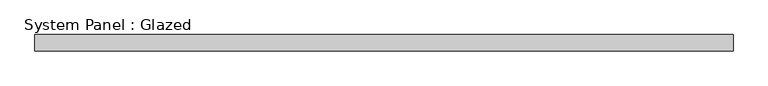
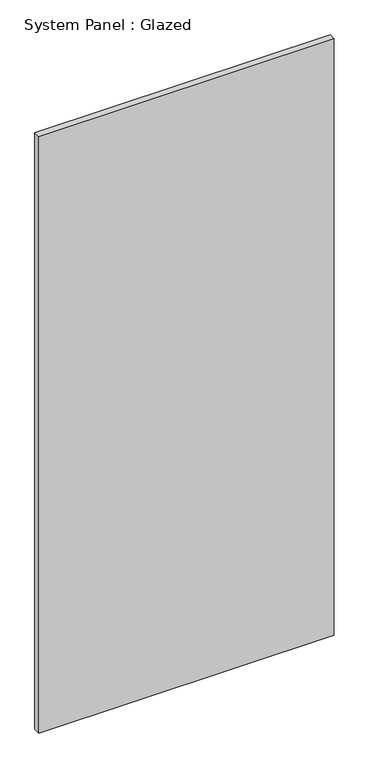
"""IFC4 building model written with IfcOpenShell, lengths in millimetres: plate geometry, System Panel : Glazed."""

from ifc_helpers import new_model, si_unit, origin, origin_with_axes, place, context, project, spatial, polyline, outline, extrude, source, transform, mapped, element, save


def system_panel_glazed_d847cfee(model_context):
    return source(origin(), model_context, "Body", "SweptSolid", [
        extrude(outline(polyline([(549.275, 19.05), (-549.275, 19.05), (-549.275, 44.45), (549.275, 44.45), (549.275, 19.05)])), origin_with_axes(), (0.0, 0.0, 1.0), 2343.15),
    ])


if __name__ == "__main__":
    model = new_model("IFC4")
    model_context = context("Model", 3, world=origin())
    ifc_project = project(units=[si_unit("LENGTHUNIT", "METRE", prefix="MILLI")], contexts=[model_context])
    site = spatial("IfcSite", under=ifc_project)
    building = spatial("IfcBuilding", under=site)
    placement = place(None, origin())
    system_panel_glazed_shape = system_panel_glazed_d847cfee(model_context)
    element("IfcPlate", 1, ObjectType="System Panel : Glazed", at=placement, inside=building, context=model_context, shape_type="MappedRepresentation", body=[
        mapped(system_panel_glazed_shape, transform((0.0, 0.0, 0.0), x_axis=(1.0, 0.0, 0.0), y_axis=(0.0, 1.0, 0.0), z_axis=(0.0, 0.0, 1.0))),
    ])
    save(model, "model.ifc")

# Revit data of these elements
# Element 1 (IfcPlate, "System Panel : Glazed")
#   Materials on its faces: "Glass"
# Materials
#   "Glass": class "Glass", colour RGB 0 128 192, transparency 0.75
